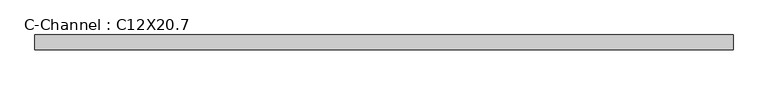
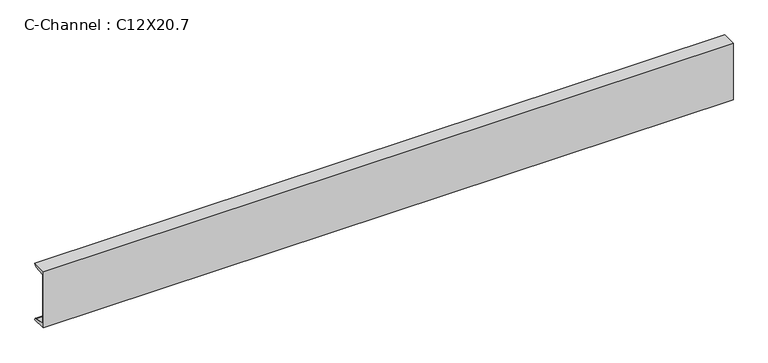
"""IFC4 building model written with IfcOpenShell, lengths in millimetres: beam geometry, C-Channel : C12X20.7."""

from ifc_helpers import new_model, si_unit, point, frame, frame_2d, origin, place, context, project, spatial, polyline, circle_curve, trimmed, segment, composite_curve, outline, extrude, source, transform, mapped, element, save


def c_channel_c12x20_7_394f2b40(model_context):
    return source(origin(), model_context, "Body", "SweptSolid", [
        extrude(outline(composite_curve([segment(polyline([(-17.7292, 152.4), (56.9468, 152.4)]), True, "CONTINUOUS"), segment(trimmed(circle_curve(frame_2d((44.2214, 152.4)), 12.7254), [point((56.9468, 152.4))], [point((44.2214, 139.6746))], False, "CARTESIAN"), True, "CONTINUOUS"), segment(polyline([(44.2214, 139.6746), (-10.5664, 130.997065), (-10.5664, -130.997065), (44.2214, -139.6746)]), True, "CONTINUOUS"), segment(trimmed(circle_curve(frame_2d((44.2214, -152.4)), 12.7254), [point((44.2214, -139.6746))], [point((56.9468, -152.4))], False, "CARTESIAN"), True, "CONTINUOUS"), segment(polyline([(56.9468, -152.4), (-17.7292, -152.4), (-17.7292, 152.4)]), True, "CONTINUOUS")], self_intersect=False)), frame((-2005.5614326, 0.0, 0.0), z_axis=(1.0, 0.0, 0.0), x_axis=(0.0, 1.0, 0.0)), (0.0, 0.0, 1.0), 3533.3717112),
    ])


if __name__ == "__main__":
    model = new_model("IFC4")
    model_context = context("Model", 3, world=origin())
    ifc_project = project(units=[si_unit("LENGTHUNIT", "METRE", prefix="MILLI")], contexts=[model_context])
    site = spatial("IfcSite", under=ifc_project)
    building = spatial("IfcBuilding", under=site)
    placement = place(None, origin())
    c_channel_c12x20_7_shape = c_channel_c12x20_7_394f2b40(model_context)
    element("IfcBeam", 1, ObjectType="C-Channel : C12X20.7", at=placement, inside=building, context=model_context, shape_type="MappedRepresentation", body=[
        mapped(c_channel_c12x20_7_shape, transform((0.0, 0.0, 0.0), x_axis=(1.0, 0.0, 0.0), y_axis=(0.0, 1.0, 0.0), z_axis=(0.0, 0.0, 1.0))),
    ])
    save(model, "model.ifc")

# Revit data of these elements
# Type "C-Channel : C12X20.7"
#   Assembly Code = "B10"
#   W = 20.7
#   Start Extension Calculation [instance default] = 10' - 0"
#   Start Extension [instance default] = -0' - 0 1/2"
#   End Extension Calculation [instance default] = 10' - 0"
#   End Extension [instance default] = -0' - 0 1/2"
#   Length [instance default] = 5' - 0"
#   bf = 0' - 2.94"
#   d = 1' - 0"
#   tf = 0' - 0.501"
#   tw = 0' - 0.282"
#   x = 0' - 0.698"
#   A = 0.0422222 SF
#   Structural Material [instance default] = Metal - Steel - ASTM A36
# Element 1 (IfcBeam, "C-Channel : C12X20.7")
#   Materials on its faces: "Metal - Steel - ASTM A36"
# Materials
#   "Metal - Steel - ASTM A36": class "Metal", colour RGB 199 199 199, transparency 0
